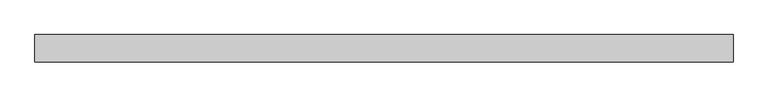
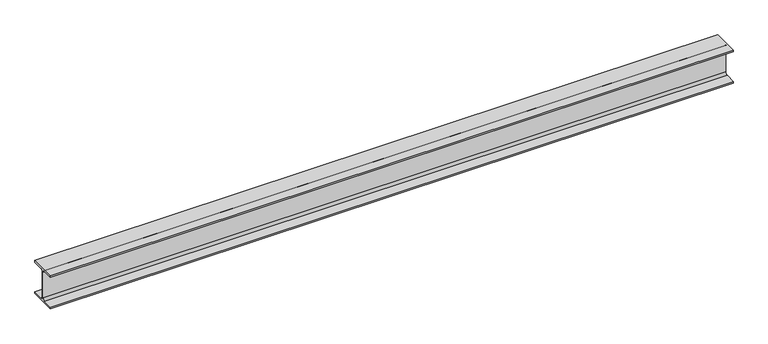
"""IFC4 building model written with IfcOpenShell, lengths in millimetres: beam geometry, 0912_Steel Framing_H-KSD3502 : H_SB_AR_S02_H-194x150x6x9_Platform."""

from ifc_helpers import new_model, si_unit, point, frame, frame_2d, origin, place, context, project, spatial, polyline, circle_curve, trimmed, segment, composite_curve, outline, extrude, source, transform, mapped, element, save


def beam_533db150(model_context):
    return source(origin(), model_context, "Body", "SweptSolid", [
        extrude(outline(composite_curve([segment(polyline([(75.0, -88.0), (75.0, -97.0), (-75.0, -97.0), (-75.0, -88.0), (-16.0, -88.0)]), True, "CONTINUOUS"), segment(trimmed(circle_curve(frame_2d((-16.0, -75.0)), 13.0), [point((-16.0, -88.0))], [point((-3.0, -75.0))], True, "CARTESIAN"), True, "CONTINUOUS"), segment(polyline([(-3.0, -75.0), (-3.0, 75.0)]), True, "CONTINUOUS"), segment(trimmed(circle_curve(frame_2d((-16.0, 75.0)), 13.0), [point((-3.0, 75.0))], [point((-16.0, 88.0))], True, "CARTESIAN"), True, "CONTINUOUS"), segment(polyline([(-16.0, 88.0), (-75.0, 88.0), (-75.0, 97.0), (75.0, 97.0), (75.0, 88.0), (16.0, 88.0)]), True, "CONTINUOUS"), segment(trimmed(circle_curve(frame_2d((16.0, 75.0)), 13.0), [point((16.0, 88.0))], [point((3.0, 75.0))], True, "CARTESIAN"), True, "CONTINUOUS"), segment(polyline([(3.0, 75.0), (3.0, -75.0)]), True, "CONTINUOUS"), segment(trimmed(circle_curve(frame_2d((16.0, -75.0)), 13.0), [point((3.0, -75.0))], [point((16.0, -88.0))], True, "CARTESIAN"), True, "CONTINUOUS"), segment(polyline([(16.0, -88.0), (75.0, -88.0)]), True, "CONTINUOUS")], self_intersect=False)), frame((-1912.3, 0.0, 0.0), z_axis=(1.0, 0.0, 0.0), x_axis=(0.0, 1.0, 0.0)), (0.0, 0.0, 1.0), 3824.6),
    ])


if __name__ == "__main__":
    model = new_model("IFC4")
    model_context = context("Model", 3, world=origin())
    ifc_project = project(units=[si_unit("LENGTHUNIT", "METRE", prefix="MILLI")], contexts=[model_context])
    site = spatial("IfcSite", under=ifc_project)
    building = spatial("IfcBuilding", under=site)
    placement = place(None, origin())
    beam_shape = beam_533db150(model_context)
    element("IfcBeam", 1, ObjectType="0912_Steel Framing_H-KSD3502 : H_SB_AR_S02_H-194x150x6x9_Platform", at=placement, inside=building, context=model_context, shape_type="MappedRepresentation", body=[
        mapped(beam_shape, transform((0.0, 0.0, 0.0), x_axis=(1.0, 0.0, 0.0), y_axis=(0.0, 1.0, 0.0), z_axis=(0.0, 0.0, 1.0))),
    ])
    save(model, "model.ifc")

# Revit data of these elements
# Type "0912_Steel Framing_H-KSD3502 : H_SB_AR_S02_H-194x150x6x9_Platform"
#   H_Q'ty Cal Type Tag = "SB-Q2"
#   H_WM Code_1 = "S01AA073-00001 |  | TON | Main Steel Structure Fabrication Work | Shelter/Building | Medium Steel - Standard |  |  |  |  |  |  | Material: (   ) | (90)KG/M>Weight≥(30)KG/M | S01AA073-00001 Main Steel Structure Fabrication Work Shelter/Building Medium Steel - Standard         | - Material: ( ASTM A36 )\n- (90)KG/M>Weight≥(30)KG/M"
#   H_WM Code_2 = "S03AA083-00001 |  | TON | Main Steel Structure Erection Work | Shelter/Building | Medium Steel |  |  |  |  |  |  | Material: (   ) | S03AA083-00001 Main Steel Structure Erection Work Shelter/Building Medium Steel         | - Material: ( ASTM A36 )"
#   H_WM Code_3 = "S01AA009-00001 |  | TON | Main Steel Structure Fabrication Work | Shelter/Building | Plates - Gusset, Stiffener, ETC | Material: (   ) | S01AA009-00001 Main Steel Structure Fabrication Work Shelter/Building Plates - Gusset, Stiffener, ETC         |"
#   H_WM Code_4 = "S41AA051-00001 |  | M2 | Steel Structure Paint Work | Shelter/Building | for Non-Fireproofed Steel Surface |  |  |  |  |  |  | Material: (   ) | S41AA051-00001 Steel Structure Paint Work Shelter/Building for Non-Fireproofed Steel Surface         |"
#   Width = 15.0 cm
#   Web Thickness = 0.6 cm
#   Web Fillet = 1.3 cm
#   Warping Constant = 43316.0 cm⁶
#   W = 0
#   Torsional Moment of Inertia = 8.622 cm⁴
#   Section Area = 39.01 cm²
#   Plastic Modulus weak axis = 104.0 cm³
#   Plastic Modulus strong axis = 309.0 cm³
#   Perimeter = 0.95 m²/m
#   Nominal Weight = 30.60 kgf/m
#   Moment of Inertia weak axis = 507.00 cm⁴
#   Moment of Inertia strong axis = 2690.00 cm⁴
#   Height = 19.4 cm
#   Flange Thickness = 0.9 cm
#   Elastic Modulus weak axis = 67.6 cm³
#   Elastic Modulus strong axis = 277.0 cm³
#   Centroid Vertical = 9.7 cm
#   Centroid Horizontal = 7.5 cm
#   Ix = 26900000
#   Length [instance default] = 1524 mm
#   Zx = 309000
#   b = 150 mm
#   h = 194 mm
#   r = 13 mm
#   s = 6 mm
#   t = 9 mm
#   A = 0.003901 m²
#   Structural Material [instance default] = Steel, 45-345
#   Assembly Code = ""
# Element 1 (IfcBeam, "0912_Steel Framing_H-KSD3502 : H_SB_AR_S02_H-194x150x6x9_Platform")
#   Materials on its faces: "Steel, 45-345"
# Materials
#   "Steel, 45-345": class "Metal", colour RGB 189 187 185, transparency 0, Description = "Steel 345 MPa", Cost = 0
